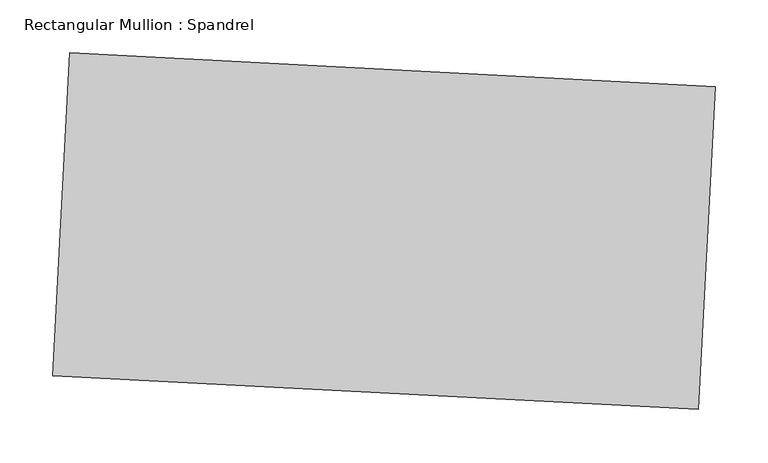
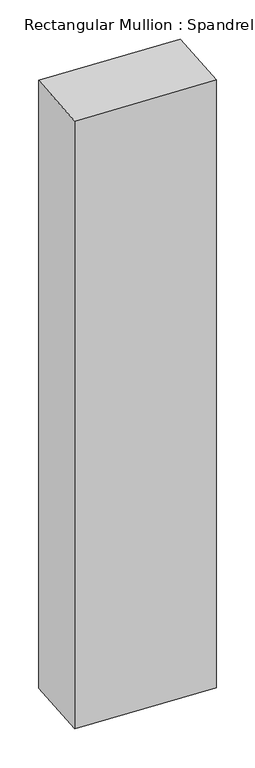
"""IFC4 building model written with IfcOpenShell, lengths in millimetres: member geometry, Rectangular Mullion : Spandrel."""

import ifcopenshell
import ifcopenshell.guid

model = None  # the IFC model being written
_history = None  # IfcOwnerHistory: only IFC2X3 demands one
_inside = {}  # id of a spatial element -> (the spatial element, [elements in it])
_under = {}  # id of a project, library or spatial element -> (it, [spatial elements below it])
_declared = {}  # id of a project -> (the project, [libraries it declares])
_typed = {}  # id of a type object -> (the type object, [elements of that type])
_made_of = {}  # id of a material, layer set ... -> (it, [elements and type objects made of it])


def new_model(schema):
    """Start an empty IFC model of exactly this schema.

    Asked for "IFC4X3", IfcOpenShell would pick the latest addendum, in which some entities
    have other attributes; the version numbers below select the first issue.
    IFC2X3 requires an IfcOwnerHistory on every rooted entity: one is made here for all.
    """
    global model, _history
    if schema == "IFC4X3":
        model = ifcopenshell.file(schema_version=(4, 3, 0, 0))
    else:
        model = ifcopenshell.file(schema=schema)
    _inside.clear()
    _under.clear()
    _declared.clear()
    _typed.clear()
    _made_of.clear()
    _history = None
    if model.schema == "IFC2X3":
        org = make("IfcOrganization", Name="unknown")
        user = make(
            "IfcPersonAndOrganization",
            ThePerson=make("IfcPerson", FamilyName="unknown"),
            TheOrganization=org,
        )
        app = make(
            "IfcApplication",
            ApplicationDeveloper=org,
            Version="unknown",
            ApplicationFullName="unknown",
            ApplicationIdentifier="unknown",
        )
        _history = make(
            "IfcOwnerHistory",
            OwningUser=user,
            OwningApplication=app,
            ChangeAction="ADDED",
            CreationDate=0,
        )
    return model


def make(cls, **values):
    """One entity of the class cls with the attributes given. An attribute that is None is left unset."""
    return model.create_entity(
        cls, **{name: value for name, value in values.items() if value is not None}
    )


def rooted(cls, **values):
    """An entity with a GlobalId (a new one), such as an element, a storey or a relation."""
    return make(cls, GlobalId=ifcopenshell.guid.new(), OwnerHistory=_history, **values)


def si_unit(unit_type, name, prefix=None):
    """IfcSIUnit, for example si_unit("LENGTHUNIT", "METRE", prefix="MILLI")."""
    return make("IfcSIUnit", UnitType=unit_type, Prefix=prefix, Name=name)


def assignment(units):
    """IfcUnitAssignment: the units of a project."""
    return None if units is None else make("IfcUnitAssignment", Units=units)


def point(xyz):
    """IfcCartesianPoint."""
    return None if xyz is None else make("IfcCartesianPoint", Coordinates=xyz)


def direction(xyz):
    """IfcDirection."""
    return None if xyz is None else make("IfcDirection", DirectionRatios=xyz)


def frame(location, z_axis=None, x_axis=None):
    """IfcAxis2Placement3D, a coordinate frame: its origin and axes. An axis left out is left unset."""
    return make(
        "IfcAxis2Placement3D",
        Location=point(location),
        Axis=direction(z_axis),
        RefDirection=direction(x_axis),
    )


def origin():
    """The frame at (0, 0, 0) with its axes left unset."""
    return frame((0.0, 0.0, 0.0))


def place(relative_to, where):
    """IfcLocalPlacement: puts the frame where relative to a parent placement (None: the world)."""
    return make(
        "IfcLocalPlacement", PlacementRelTo=relative_to, RelativePlacement=where
    )


def context(
    kind, dimensions, precision=None, world=None, true_north=None, identifier=None
):
    """IfcGeometricRepresentationContext, for example the 3D "Model" context."""
    return make(
        "IfcGeometricRepresentationContext",
        ContextIdentifier=identifier,
        ContextType=kind,
        CoordinateSpaceDimension=dimensions,
        Precision=precision,
        WorldCoordinateSystem=world,
        TrueNorth=true_north,
    )


def project(units=None, contexts=None):
    """IfcProject with its units and contexts."""
    return rooted(
        "IfcProject",
        Name="project",
        RepresentationContexts=contexts,
        UnitsInContext=assignment(units),
    )


def spatial(cls, under=None, at=None, **own):
    """A site, building, storey or space (cls), placed at a placement, below another one or the project."""
    s = rooted(cls, ObjectPlacement=at, **own)
    if under is not None:
        _under.setdefault(under.id(), (under, []))[1].append(s)
    return s


def polyline(points):
    """IfcPolyline through the points."""
    return make("IfcPolyline", Points=[point(p) for p in points])


def outline(outer, holes=None, kind="AREA"):
    """IfcArbitraryClosedProfileDef: a profile drawn as a closed curve; with holes, ...WithVoids."""
    if holes is None:
        return make("IfcArbitraryClosedProfileDef", ProfileType=kind, OuterCurve=outer)
    return make(
        "IfcArbitraryProfileDefWithVoids",
        ProfileType=kind,
        OuterCurve=outer,
        InnerCurves=holes,
    )


def extrude(swept, where, along, depth):
    """IfcExtrudedAreaSolid: the profile swept, set in the frame where, extruded along a direction by depth."""
    return make(
        "IfcExtrudedAreaSolid",
        SweptArea=swept,
        Position=where,
        ExtrudedDirection=direction(along),
        Depth=depth,
    )


def shape(context_of_items, identifier, shape_type, items):
    """IfcShapeRepresentation: the items that make up one representation, for example the "Body"."""
    return make(
        "IfcShapeRepresentation",
        ContextOfItems=context_of_items,
        RepresentationIdentifier=identifier,
        RepresentationType=shape_type,
        Items=items,
    )


def source(mapping_origin, context_of_items, identifier, shape_type, items):
    """IfcRepresentationMap: a shape defined once, which mapped items show again and again."""
    return make(
        "IfcRepresentationMap",
        MappingOrigin=mapping_origin,
        MappedRepresentation=shape(context_of_items, identifier, shape_type, items),
    )


def transform(
    local_origin,
    x_axis=None,
    y_axis=None,
    z_axis=None,
    scale=None,
    scale2=None,
    scale3=None,
    uniform=True,
):
    """IfcCartesianTransformationOperator3D, or its non-uniform kind. x_axis, y_axis, z_axis: its Axis1, 2, 3."""
    if uniform:
        return make(
            "IfcCartesianTransformationOperator3D",
            Axis1=direction(x_axis),
            Axis2=direction(y_axis),
            LocalOrigin=point(local_origin),
            Scale=scale,
            Axis3=direction(z_axis),
        )
    return make(
        "IfcCartesianTransformationOperator3DnonUniform",
        Axis1=direction(x_axis),
        Axis2=direction(y_axis),
        LocalOrigin=point(local_origin),
        Scale=scale,
        Axis3=direction(z_axis),
        Scale2=scale2,
        Scale3=scale3,
    )


def mapped(mapping_source, mapping_target):
    """IfcMappedItem: shows the shape of a source again, moved by a transform."""
    return make(
        "IfcMappedItem", MappingSource=mapping_source, MappingTarget=mapping_target
    )


def made_of(thing, what):
    """Note that an element or type object is made of a material, layer set ...; save() writes the relation."""
    if what is not None:
        _made_of.setdefault(what.id(), (what, []))[1].append(thing)
    return thing


def element(
    cls,
    number,
    at=None,
    inside=None,
    cuts=None,
    type_object=None,
    material=None,
    context=None,
    identifier="Body",
    shape_type=None,
    held_by="IfcProductDefinitionShape",
    body=None,
    shapes=None,
    **own,
):
    """One element of the class cls, such as IfcWall. Its Tag is "e" and its number.

    at: its placement. inside: the storey or other place that contains it. cuts: it is an
    opening in that element (IfcRelVoidsElement). A single representation is given by context,
    identifier, shape_type and body (its items); several are given by shapes. held_by: the class
    of the entity that holds the representations. save() writes the other relations.
    """
    e = rooted(cls, Tag="e%d" % number, ObjectPlacement=at, **own)
    if body is not None:
        shapes = [shape(context, identifier, shape_type, body)]
    if shapes is not None:
        e.Representation = make(held_by, Representations=shapes)
    if inside is not None:
        _inside.setdefault(inside.id(), (inside, []))[1].append(e)
    if cuts is not None:
        rooted(
            "IfcRelVoidsElement", RelatingBuildingElement=cuts, RelatedOpeningElement=e
        )
    if type_object is not None:
        _typed.setdefault(type_object.id(), (type_object, []))[1].append(e)
    return made_of(e, material)


def aggregate(whole, parts):
    """IfcRelAggregates: a whole, such as a stair, and the parts it consists of."""
    return rooted("IfcRelAggregates", RelatingObject=whole, RelatedObjects=parts)


def save(model, path):
    """Write the relations noted so far, then the file.

    IfcRelAggregates (storeys below a building ...), IfcRelContainedInSpatialStructure (elements
    in a storey), IfcRelDefinesByType, IfcRelAssociatesMaterial and IfcRelDeclares: one each for
    every whole, place, type object, material and project.
    """
    for whole, parts in _under.values():
        aggregate(whole, parts)
    for where, things in _inside.values():
        rooted(
            "IfcRelContainedInSpatialStructure",
            RelatedElements=things,
            RelatingStructure=where,
        )
    for kind, things in _typed.values():
        rooted("IfcRelDefinesByType", RelatedObjects=things, RelatingType=kind)
    for what, things in _made_of.values():
        rooted("IfcRelAssociatesMaterial", RelatedObjects=things, RelatingMaterial=what)
    for by, libraries in _declared.values():
        rooted("IfcRelDeclares", RelatingContext=by, RelatedDefinitions=libraries)
    model.write(path)


def rectangular_mullion_spandrel_ffee690b(model_context):
    return source(origin(), model_context, "Body", "SweptSolid", [
        extrude(outline(polyline([(7.5582819, 136.2391416), (-8.3937175, -168.1431406), (-617.1582819, -136.2391416), (-601.2062825, 168.1431406), (7.5582819, 136.2391416)])), frame((0.0, 0.0, -2845.3134854), z_axis=(0.0, 0.0, 1.0), x_axis=(1.0, 0.0, 0.0)), (0.0, 0.0, 1.0), 2845.3134854),
    ])


if __name__ == "__main__":
    model = new_model("IFC4")
    model_context = context("Model", 3, world=origin())
    ifc_project = project(units=[si_unit("LENGTHUNIT", "METRE", prefix="MILLI")], contexts=[model_context])
    site = spatial("IfcSite", under=ifc_project)
    building = spatial("IfcBuilding", under=site)
    placement = place(None, origin())
    rectangular_mullion_spandrel_shape = rectangular_mullion_spandrel_ffee690b(model_context)
    element("IfcMember", 1, ObjectType="Rectangular Mullion : Spandrel", at=placement, inside=building, context=model_context, shape_type="MappedRepresentation", body=[
        mapped(rectangular_mullion_spandrel_shape, transform((0.0, 0.0, 0.0), x_axis=(1.0, 0.0, 0.0), y_axis=(0.0, 1.0, 0.0), z_axis=(0.0, 0.0, 1.0))),
    ])
    save(model, "model.ifc")

# Revit data of these elements
# Type "Rectangular Mullion : Spandrel"
#   built-in parameter 1007304 = 1 (stored number, unit not read)
#   built-in parameter 1007301 = 1 (stored number, unit not read)
#   built-in parameter 1007300 = 1 (stored number, unit not read)
# Element 1 (IfcMember, "Rectangular Mullion : Spandrel")
#   Materials on its faces: "Aluminum"
# Materials
#   "Aluminum": class "Metal", colour RGB 247 247 247, transparency 0, Description = "Aluminum 6061", Cost = 0
